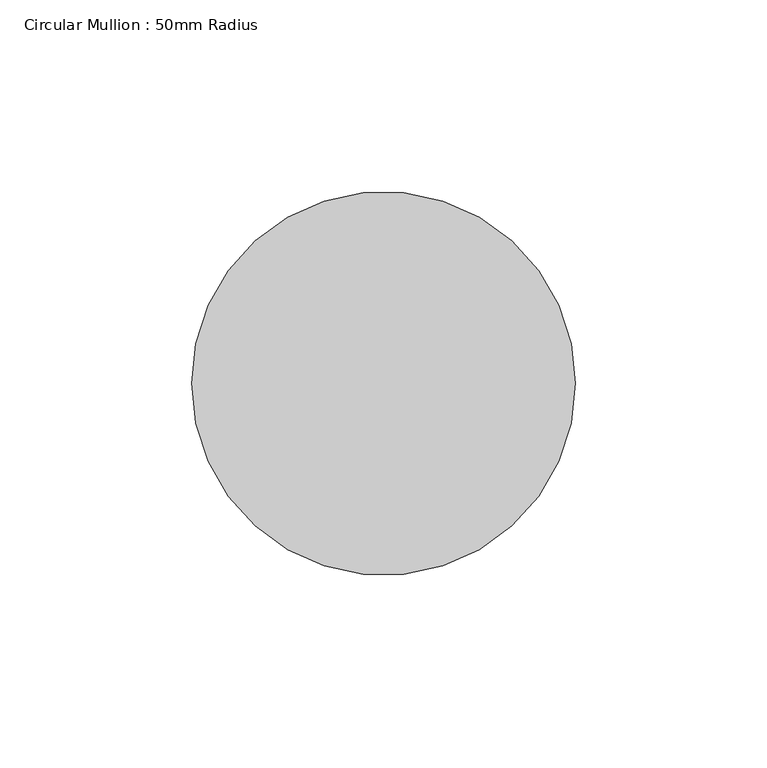
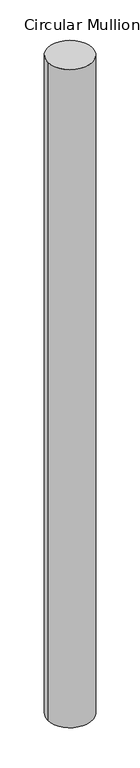
"""IFC4 building model written with IfcOpenShell, lengths in millimetres: member geometry, Circular Mullion : 50mm Radius."""

from ifc_helpers import new_model, si_unit, point, frame, origin, origin_2d, place, context, project, spatial, circle_curve, trimmed, segment, composite_curve, outline, extrude, source, transform, mapped, element, save


def circular_mullion_50mm_radius_b20b040d(model_context):
    return source(origin(), model_context, "Body", "SweptSolid", [
        extrude(outline(composite_curve([segment(trimmed(circle_curve(origin_2d(), 50.0), [point((50.0, 0.0))], [point((-50.0, 0.0))], False, "CARTESIAN"), True, "CONTINUOUS"), segment(trimmed(circle_curve(origin_2d(), 50.0), [point((-50.0, 0.0))], [point((50.0, 0.0))], False, "CARTESIAN"), True, "CONTINUOUS")], self_intersect=False)), frame((0.0, 0.0, -1563.8843459), z_axis=(0.0, 0.0, 1.0), x_axis=(1.0, 0.0, 0.0)), (0.0, 0.0, 1.0), 1563.8843459),
    ])


if __name__ == "__main__":
    model = new_model("IFC4")
    model_context = context("Model", 3, world=origin())
    ifc_project = project(units=[si_unit("LENGTHUNIT", "METRE", prefix="MILLI")], contexts=[model_context])
    site = spatial("IfcSite", under=ifc_project)
    building = spatial("IfcBuilding", under=site)
    placement = place(None, origin())
    circular_mullion_50mm_radius_shape = circular_mullion_50mm_radius_b20b040d(model_context)
    element("IfcMember", 1, ObjectType="Circular Mullion : 50mm Radius", at=placement, inside=building, context=model_context, shape_type="MappedRepresentation", body=[
        mapped(circular_mullion_50mm_radius_shape, transform((0.0, 0.0, 0.0), x_axis=(1.0, 0.0, 0.0), y_axis=(0.0, 1.0, 0.0), z_axis=(0.0, 0.0, 1.0))),
    ])
    save(model, "model.ifc")

# Revit data of these elements
# Type "Circular Mullion : 50mm Radius"
#   built-in parameter 1007350 = 0.164042 (stored number, unit not read)
# Element 1 (IfcMember, "Circular Mullion : 50mm Radius")
#   Materials on its faces: "Aluminium"
# Materials
#   "Aluminium": class "Metal", colour RGB 247 247 247, transparency 0, Description = "Aluminium 6061", Cost = 0
